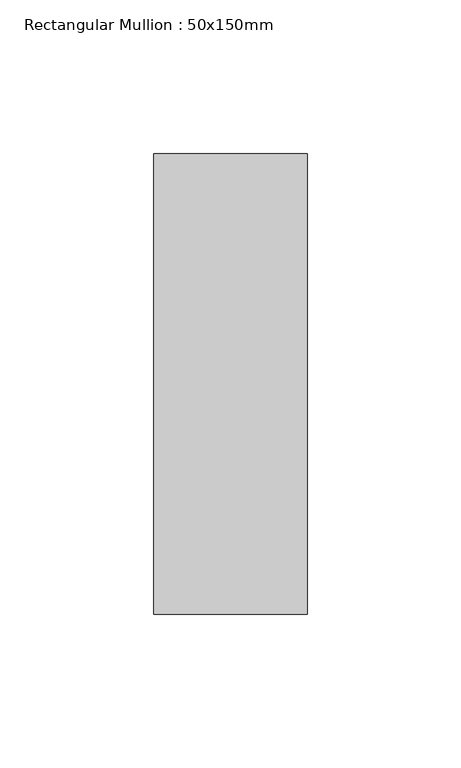
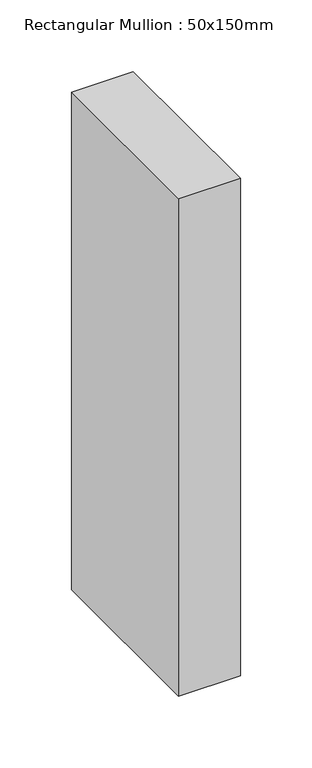
"""IFC4 building model written with IfcOpenShell, lengths in millimetres: member geometry, Rectangular Mullion : 50x150mm."""

from ifc_helpers import new_model, si_unit, frame, origin, place, context, project, spatial, polyline, outline, extrude, source, transform, mapped, element, save


def rectangular_mullion_50x150mm_89c22e8d(model_context):
    return source(origin(), model_context, "Body", "SweptSolid", [
        extrude(outline(polyline([(0.0, 75.0), (0.0, -75.0), (-50.0, -75.0), (-50.0, 75.0), (0.0, 75.0)])), frame((0.0, 0.0, -425.0), z_axis=(0.0, 0.0, 1.0), x_axis=(1.0, 0.0, 0.0)), (0.0, 0.0, 1.0), 425.0),
    ])


if __name__ == "__main__":
    model = new_model("IFC4")
    model_context = context("Model", 3, world=origin())
    ifc_project = project(units=[si_unit("LENGTHUNIT", "METRE", prefix="MILLI")], contexts=[model_context])
    site = spatial("IfcSite", under=ifc_project)
    building = spatial("IfcBuilding", under=site)
    placement = place(None, origin())
    rectangular_mullion_50x150mm_shape = rectangular_mullion_50x150mm_89c22e8d(model_context)
    element("IfcMember", 1, ObjectType="Rectangular Mullion : 50x150mm", at=placement, inside=building, context=model_context, shape_type="MappedRepresentation", body=[
        mapped(rectangular_mullion_50x150mm_shape, transform((0.0, 0.0, 0.0), x_axis=(1.0, 0.0, 0.0), y_axis=(0.0, 1.0, 0.0), z_axis=(0.0, 0.0, 1.0))),
    ])
    save(model, "model.ifc")

# Revit data of these elements
# Type "Rectangular Mullion : 50x150mm"
#   Keynote = "H11"
#   built-in parameter 1007304 = 0.492126 (stored number, unit not read)
#   built-in parameter 1007301 = 0.082021 (stored number, unit not read)
#   built-in parameter 1007300 = 0.082021 (stored number, unit not read)
# Element 1 (IfcMember, "Rectangular Mullion : 50x150mm")
#   Materials on its faces: "Aluminium"
# Materials
#   "Aluminium": class "Metal", colour RGB 247 247 247, transparency 0, Description = "Aluminium 6061", Cost = 0
